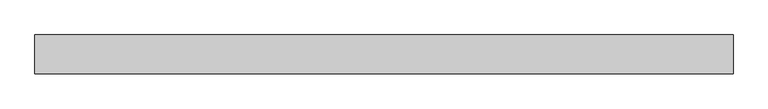
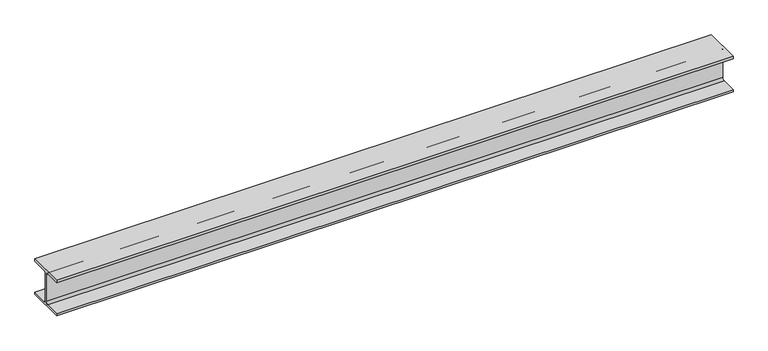
"""IFC4 building model written with IfcOpenShell, lengths in millimetres: beam geometry, 0912_Steel Framing_H-KSD3502 : H_SB_ASB_H-200x200x8x12."""

import ifcopenshell
import ifcopenshell.guid

model = None  # the IFC model being written
_history = None  # IfcOwnerHistory: only IFC2X3 demands one
_inside = {}  # id of a spatial element -> (the spatial element, [elements in it])
_under = {}  # id of a project, library or spatial element -> (it, [spatial elements below it])
_declared = {}  # id of a project -> (the project, [libraries it declares])
_typed = {}  # id of a type object -> (the type object, [elements of that type])
_made_of = {}  # id of a material, layer set ... -> (it, [elements and type objects made of it])


def new_model(schema):
    """Start an empty IFC model of exactly this schema.

    Asked for "IFC4X3", IfcOpenShell would pick the latest addendum, in which some entities
    have other attributes; the version numbers below select the first issue.
    IFC2X3 requires an IfcOwnerHistory on every rooted entity: one is made here for all.
    """
    global model, _history
    if schema == "IFC4X3":
        model = ifcopenshell.file(schema_version=(4, 3, 0, 0))
    else:
        model = ifcopenshell.file(schema=schema)
    _inside.clear()
    _under.clear()
    _declared.clear()
    _typed.clear()
    _made_of.clear()
    _history = None
    if model.schema == "IFC2X3":
        org = make("IfcOrganization", Name="unknown")
        user = make(
            "IfcPersonAndOrganization",
            ThePerson=make("IfcPerson", FamilyName="unknown"),
            TheOrganization=org,
        )
        app = make(
            "IfcApplication",
            ApplicationDeveloper=org,
            Version="unknown",
            ApplicationFullName="unknown",
            ApplicationIdentifier="unknown",
        )
        _history = make(
            "IfcOwnerHistory",
            OwningUser=user,
            OwningApplication=app,
            ChangeAction="ADDED",
            CreationDate=0,
        )
    return model


def make(cls, **values):
    """One entity of the class cls with the attributes given. An attribute that is None is left unset."""
    return model.create_entity(
        cls, **{name: value for name, value in values.items() if value is not None}
    )


def rooted(cls, **values):
    """An entity with a GlobalId (a new one), such as an element, a storey or a relation."""
    return make(cls, GlobalId=ifcopenshell.guid.new(), OwnerHistory=_history, **values)


def si_unit(unit_type, name, prefix=None):
    """IfcSIUnit, for example si_unit("LENGTHUNIT", "METRE", prefix="MILLI")."""
    return make("IfcSIUnit", UnitType=unit_type, Prefix=prefix, Name=name)


def assignment(units):
    """IfcUnitAssignment: the units of a project."""
    return None if units is None else make("IfcUnitAssignment", Units=units)


def point(xyz):
    """IfcCartesianPoint."""
    return None if xyz is None else make("IfcCartesianPoint", Coordinates=xyz)


def direction(xyz):
    """IfcDirection."""
    return None if xyz is None else make("IfcDirection", DirectionRatios=xyz)


def frame(location, z_axis=None, x_axis=None):
    """IfcAxis2Placement3D, a coordinate frame: its origin and axes. An axis left out is left unset."""
    return make(
        "IfcAxis2Placement3D",
        Location=point(location),
        Axis=direction(z_axis),
        RefDirection=direction(x_axis),
    )


def frame_2d(location, x_axis=None):
    """IfcAxis2Placement2D, a coordinate frame in the plane: its origin and x axis."""
    return make(
        "IfcAxis2Placement2D", Location=point(location), RefDirection=direction(x_axis)
    )


def origin():
    """The frame at (0, 0, 0) with its axes left unset."""
    return frame((0.0, 0.0, 0.0))


def place(relative_to, where):
    """IfcLocalPlacement: puts the frame where relative to a parent placement (None: the world)."""
    return make(
        "IfcLocalPlacement", PlacementRelTo=relative_to, RelativePlacement=where
    )


def context(
    kind, dimensions, precision=None, world=None, true_north=None, identifier=None
):
    """IfcGeometricRepresentationContext, for example the 3D "Model" context."""
    return make(
        "IfcGeometricRepresentationContext",
        ContextIdentifier=identifier,
        ContextType=kind,
        CoordinateSpaceDimension=dimensions,
        Precision=precision,
        WorldCoordinateSystem=world,
        TrueNorth=true_north,
    )


def project(units=None, contexts=None):
    """IfcProject with its units and contexts."""
    return rooted(
        "IfcProject",
        Name="project",
        RepresentationContexts=contexts,
        UnitsInContext=assignment(units),
    )


def spatial(cls, under=None, at=None, **own):
    """A site, building, storey or space (cls), placed at a placement, below another one or the project."""
    s = rooted(cls, ObjectPlacement=at, **own)
    if under is not None:
        _under.setdefault(under.id(), (under, []))[1].append(s)
    return s


def polyline(points):
    """IfcPolyline through the points."""
    return make("IfcPolyline", Points=[point(p) for p in points])


def circle_curve(where, radius):
    """IfcCircle in the frame where."""
    return make("IfcCircle", Position=where, Radius=radius)


def trimmed(basis, trim1, trim2, sense, master):
    """IfcTrimmedCurve: the piece of a basis curve between two trims."""
    return make(
        "IfcTrimmedCurve",
        BasisCurve=basis,
        Trim1=trim1,
        Trim2=trim2,
        SenseAgreement=sense,
        MasterRepresentation=master,
    )


def segment(curve, same_sense, transition):
    """IfcCompositeCurveSegment."""
    return make(
        "IfcCompositeCurveSegment",
        Transition=transition,
        SameSense=same_sense,
        ParentCurve=curve,
    )


def composite_curve(segments, self_intersect=None):
    """IfcCompositeCurve: segments joined end to end."""
    return make("IfcCompositeCurve", Segments=segments, SelfIntersect=self_intersect)


def outline(outer, holes=None, kind="AREA"):
    """IfcArbitraryClosedProfileDef: a profile drawn as a closed curve; with holes, ...WithVoids."""
    if holes is None:
        return make("IfcArbitraryClosedProfileDef", ProfileType=kind, OuterCurve=outer)
    return make(
        "IfcArbitraryProfileDefWithVoids",
        ProfileType=kind,
        OuterCurve=outer,
        InnerCurves=holes,
    )


def extrude(swept, where, along, depth):
    """IfcExtrudedAreaSolid: the profile swept, set in the frame where, extruded along a direction by depth."""
    return make(
        "IfcExtrudedAreaSolid",
        SweptArea=swept,
        Position=where,
        ExtrudedDirection=direction(along),
        Depth=depth,
    )


def shape(context_of_items, identifier, shape_type, items):
    """IfcShapeRepresentation: the items that make up one representation, for example the "Body"."""
    return make(
        "IfcShapeRepresentation",
        ContextOfItems=context_of_items,
        RepresentationIdentifier=identifier,
        RepresentationType=shape_type,
        Items=items,
    )


def source(mapping_origin, context_of_items, identifier, shape_type, items):
    """IfcRepresentationMap: a shape defined once, which mapped items show again and again."""
    return make(
        "IfcRepresentationMap",
        MappingOrigin=mapping_origin,
        MappedRepresentation=shape(context_of_items, identifier, shape_type, items),
    )


def transform(
    local_origin,
    x_axis=None,
    y_axis=None,
    z_axis=None,
    scale=None,
    scale2=None,
    scale3=None,
    uniform=True,
):
    """IfcCartesianTransformationOperator3D, or its non-uniform kind. x_axis, y_axis, z_axis: its Axis1, 2, 3."""
    if uniform:
        return make(
            "IfcCartesianTransformationOperator3D",
            Axis1=direction(x_axis),
            Axis2=direction(y_axis),
            LocalOrigin=point(local_origin),
            Scale=scale,
            Axis3=direction(z_axis),
        )
    return make(
        "IfcCartesianTransformationOperator3DnonUniform",
        Axis1=direction(x_axis),
        Axis2=direction(y_axis),
        LocalOrigin=point(local_origin),
        Scale=scale,
        Axis3=direction(z_axis),
        Scale2=scale2,
        Scale3=scale3,
    )


def mapped(mapping_source, mapping_target):
    """IfcMappedItem: shows the shape of a source again, moved by a transform."""
    return make(
        "IfcMappedItem", MappingSource=mapping_source, MappingTarget=mapping_target
    )


def made_of(thing, what):
    """Note that an element or type object is made of a material, layer set ...; save() writes the relation."""
    if what is not None:
        _made_of.setdefault(what.id(), (what, []))[1].append(thing)
    return thing


def element(
    cls,
    number,
    at=None,
    inside=None,
    cuts=None,
    type_object=None,
    material=None,
    context=None,
    identifier="Body",
    shape_type=None,
    held_by="IfcProductDefinitionShape",
    body=None,
    shapes=None,
    **own,
):
    """One element of the class cls, such as IfcWall. Its Tag is "e" and its number.

    at: its placement. inside: the storey or other place that contains it. cuts: it is an
    opening in that element (IfcRelVoidsElement). A single representation is given by context,
    identifier, shape_type and body (its items); several are given by shapes. held_by: the class
    of the entity that holds the representations. save() writes the other relations.
    """
    e = rooted(cls, Tag="e%d" % number, ObjectPlacement=at, **own)
    if body is not None:
        shapes = [shape(context, identifier, shape_type, body)]
    if shapes is not None:
        e.Representation = make(held_by, Representations=shapes)
    if inside is not None:
        _inside.setdefault(inside.id(), (inside, []))[1].append(e)
    if cuts is not None:
        rooted(
            "IfcRelVoidsElement", RelatingBuildingElement=cuts, RelatedOpeningElement=e
        )
    if type_object is not None:
        _typed.setdefault(type_object.id(), (type_object, []))[1].append(e)
    return made_of(e, material)


def aggregate(whole, parts):
    """IfcRelAggregates: a whole, such as a stair, and the parts it consists of."""
    return rooted("IfcRelAggregates", RelatingObject=whole, RelatedObjects=parts)


def save(model, path):
    """Write the relations noted so far, then the file.

    IfcRelAggregates (storeys below a building ...), IfcRelContainedInSpatialStructure (elements
    in a storey), IfcRelDefinesByType, IfcRelAssociatesMaterial and IfcRelDeclares: one each for
    every whole, place, type object, material and project.
    """
    for whole, parts in _under.values():
        aggregate(whole, parts)
    for where, things in _inside.values():
        rooted(
            "IfcRelContainedInSpatialStructure",
            RelatedElements=things,
            RelatingStructure=where,
        )
    for kind, things in _typed.values():
        rooted("IfcRelDefinesByType", RelatedObjects=things, RelatingType=kind)
    for what, things in _made_of.values():
        rooted("IfcRelAssociatesMaterial", RelatedObjects=things, RelatingMaterial=what)
    for by, libraries in _declared.values():
        rooted("IfcRelDeclares", RelatingContext=by, RelatedDefinitions=libraries)
    model.write(path)


def beam_c0af7261(model_context):
    return source(origin(), model_context, "Body", "SweptSolid", [
        extrude(outline(composite_curve([segment(polyline([(100.0, -88.0), (100.0, -100.0), (-100.0, -100.0), (-100.0, -88.0), (-17.0, -88.0)]), True, "CONTINUOUS"), segment(trimmed(circle_curve(frame_2d((-17.0, -75.0)), 13.0), [point((-17.0, -88.0))], [point((-4.0, -75.0))], True, "CARTESIAN"), True, "CONTINUOUS"), segment(polyline([(-4.0, -75.0), (-4.0, 75.0)]), True, "CONTINUOUS"), segment(trimmed(circle_curve(frame_2d((-17.0, 75.0)), 13.0), [point((-4.0, 75.0))], [point((-17.0, 88.0))], True, "CARTESIAN"), True, "CONTINUOUS"), segment(polyline([(-17.0, 88.0), (-100.0, 88.0), (-100.0, 100.0), (100.0, 100.0), (100.0, 88.0), (17.0, 88.0)]), True, "CONTINUOUS"), segment(trimmed(circle_curve(frame_2d((17.0, 75.0)), 13.0), [point((17.0, 88.0))], [point((4.0, 75.0))], True, "CARTESIAN"), True, "CONTINUOUS"), segment(polyline([(4.0, 75.0), (4.0, -75.0)]), True, "CONTINUOUS"), segment(trimmed(circle_curve(frame_2d((17.0, -75.0)), 13.0), [point((4.0, -75.0))], [point((17.0, -88.0))], True, "CARTESIAN"), True, "CONTINUOUS"), segment(polyline([(17.0, -88.0), (100.0, -88.0)]), True, "CONTINUOUS")], self_intersect=False)), frame((-1668.0611839, 0.0, 0.0), z_axis=(1.0, 0.0, 0.0), x_axis=(0.0, 1.0, 0.0)), (0.0, 0.0, 1.0), 3604.1166019),
    ])


if __name__ == "__main__":
    model = new_model("IFC4")
    model_context = context("Model", 3, world=origin())
    ifc_project = project(units=[si_unit("LENGTHUNIT", "METRE", prefix="MILLI")], contexts=[model_context])
    site = spatial("IfcSite", under=ifc_project)
    building = spatial("IfcBuilding", under=site)
    placement = place(None, origin())
    beam_shape = beam_c0af7261(model_context)
    element("IfcBeam", 1, ObjectType="0912_Steel Framing_H-KSD3502 : H_SB_ASB_H-200x200x8x12", at=placement, inside=building, context=model_context, shape_type="MappedRepresentation", body=[
        mapped(beam_shape, transform((0.0, 0.0, 0.0), x_axis=(1.0, 0.0, 0.0), y_axis=(0.0, 1.0, 0.0), z_axis=(0.0, 0.0, 1.0))),
    ])
    save(model, "model.ifc")

# Revit data of these elements
# Type "0912_Steel Framing_H-KSD3502 : H_SB_ASB_H-200x200x8x12"
#   H_WM Code_1 = "S01AA002-00001 | Main Steel Structure Fabrication Work | Shelter/Building | Medium Steel - Standard (90KG/M>Weight≥30KG/M) | Material: (   )"
#   H_WM Code_2 = "S03AA028-00001 | Main Steel Structure Erection Work | Shelter/Building | Medium Steel (90KG/M>Weight≥30KG/M) | Material: (   )"
#   H_WM Code_3 = "S01AA010-00001 | Main Steel Structure Fabrication Work | Shelter/Building | Steel Painting/Coating | for Non-Fireproofed Steel Surface, Surface Preparation, Primer, Second & Final Coat | Material: (   )"
#   H_Q'ty Cal Type Tag = "SB-Q2"
#   Width = 20.0 cm
#   Web Thickness = 0.8 cm
#   Web Fillet = 1.3 cm
#   Warping Constant = 141000.0 cm⁶
#   W = 0
#   Torsional Moment of Inertia = 26.2485 cm⁴
#   Section Area = 63.53 cm²
#   Plastic Modulus weak axis = 244.0 cm³
#   Plastic Modulus strong axis = 525.0 cm³
#   Perimeter = 1.16 m²/m
#   Nominal Weight = 49.90 kgf/m
#   Moment of Inertia weak axis = 1600.00 cm⁴
#   Moment of Inertia strong axis = 4720.00 cm⁴
#   Height = 20.0 cm
#   Flange Thickness = 1.2 cm
#   Elastic Modulus weak axis = 160.0 cm³
#   Elastic Modulus strong axis = 472.0 cm³
#   Centroid Vertical = 10.0 cm
#   Centroid Horizontal = 10.0 cm
#   Ix = 47200000
#   Length [instance default] = 1.5240 m
#   Zx = 525000
#   b = 0.2000 m
#   h = 0.2000 m
#   r = 0.0130 m
#   s = 0.0080 m
#   t = 0.0120 m
#   A = 0.006353 m²
#   Structural Material [instance default] = Steel, 45-345
#   Assembly Code = ""
# Element 1 (IfcBeam, "0912_Steel Framing_H-KSD3502 : H_SB_ASB_H-200x200x8x12")
#   Structural Material = none
# Materials
#   "Steel, 45-345": class "Metal", colour RGB 189 187 185, transparency 0, Description = "Steel 345 MPa", Cost = 0
